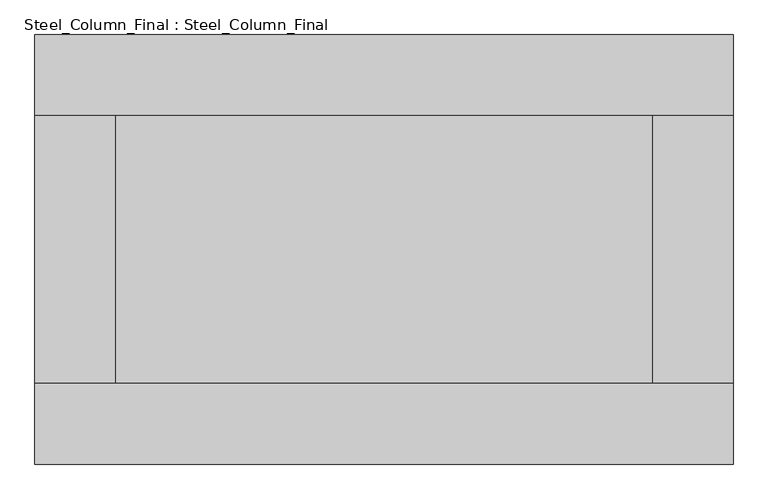
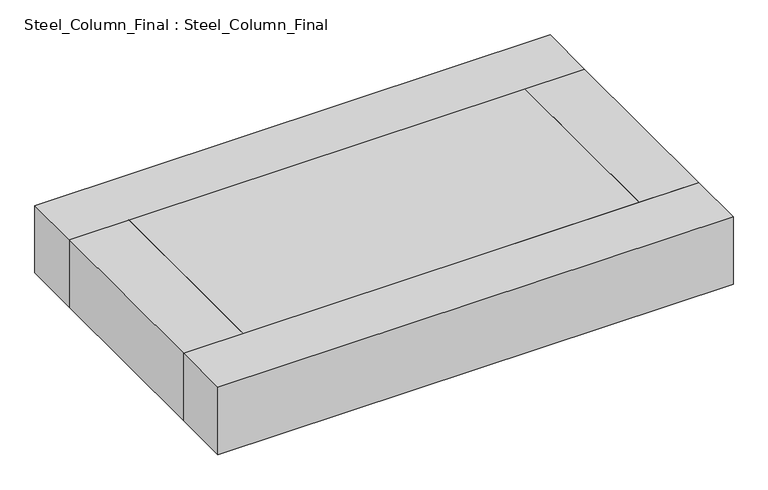
"""IFC4 building model written with IfcOpenShell, lengths in millimetres: proxy geometry, Steel_Column_Final : Steel_Column_Final."""

from ifc_helpers import new_model, si_unit, frame, origin, place, context, project, spatial, polyline, outline, extrude, source, transform, mapped, element, save


def steel_column_final_steel_column_final_5115e00a(model_context):
    return source(origin(), model_context, "Body", "SweptSolid", [
        extrude(outline(polyline([(6500.0, 2500.0), (-6500.0, 2500.0), (-6500.0, 4000.0), (6500.0, 4000.0), (6500.0, 2500.0)])), frame((0.0, 0.0, 43700.0), z_axis=(0.0, 0.0, 1.0), x_axis=(1.0, 0.0, 0.0)), (0.0, 0.0, 1.0), 1800.0),
        extrude(outline(polyline([(-6500.0, -2500.0), (6500.0, -2500.0), (6500.0, -4000.0), (-6500.0, -4000.0), (-6500.0, -2500.0)])), frame((0.0, 0.0, 43700.0), z_axis=(0.0, 0.0, 1.0), x_axis=(1.0, 0.0, 0.0)), (0.0, 0.0, 1.0), 1800.0),
        extrude(outline(polyline([(5000.0, -2500.0), (5000.0, 2500.0), (6500.0, 2500.0), (6500.0, -2500.0), (5000.0, -2500.0)])), frame((0.0, 0.0, 43700.0), z_axis=(0.0, 0.0, 1.0), x_axis=(1.0, 0.0, 0.0)), (0.0, 0.0, 1.0), 1800.0),
        extrude(outline(polyline([(-5000.0, 2500.0), (-5000.0, -2500.0), (-6500.0, -2500.0), (-6500.0, 2500.0), (-5000.0, 2500.0)])), frame((0.0, 0.0, 43700.0), z_axis=(0.0, 0.0, 1.0), x_axis=(1.0, 0.0, 0.0)), (0.0, 0.0, 1.0), 1800.0),
        extrude(outline(polyline([(-5000.0, -2500.0), (-5000.0, 2500.0), (5000.0, 2500.0), (5000.0, -2500.0), (-5000.0, -2500.0)])), frame((0.0, 0.0, 43700.0), z_axis=(0.0, 0.0, 1.0), x_axis=(1.0, 0.0, 0.0)), (0.0, 0.0, 1.0), 1800.0),
    ])


if __name__ == "__main__":
    model = new_model("IFC4")
    model_context = context("Model", 3, world=origin())
    ifc_project = project(units=[si_unit("LENGTHUNIT", "METRE", prefix="MILLI")], contexts=[model_context])
    site = spatial("IfcSite", under=ifc_project)
    building = spatial("IfcBuilding", under=site)
    placement = place(None, origin())
    steel_column_final_steel_column_final_shape = steel_column_final_steel_column_final_5115e00a(model_context)
    element("IfcBuildingElementProxy", 1, Name="Steel_Column_Final : Steel_Column_Final", ObjectType="Steel_Column_Final : Steel_Column_Final", at=placement, inside=building, context=model_context, shape_type="MappedRepresentation", body=[
        mapped(steel_column_final_steel_column_final_shape, transform((0.0, 0.0, 0.0), x_axis=(1.0, 0.0, 0.0), y_axis=(0.0, 1.0, 0.0), z_axis=(0.0, 0.0, 1.0))),
    ])
    save(model, "model.ifc")

# Revit data of these elements
# Type "Steel_Column_Final : Steel_Column_Final"
#   Top Width [instance default] = 5000 mm
#   Top Length = 10000 mm
#   Length = 21000 mm
#   Height [instance default] = 50000 mm
#   Bottom Width [instance default] = 5000 mm
#   Default Elevation = 0
# Element 1 (IfcBuildingElementProxy, "Steel_Column_Final : Steel_Column_Final")
#   Height = 43700 mm
